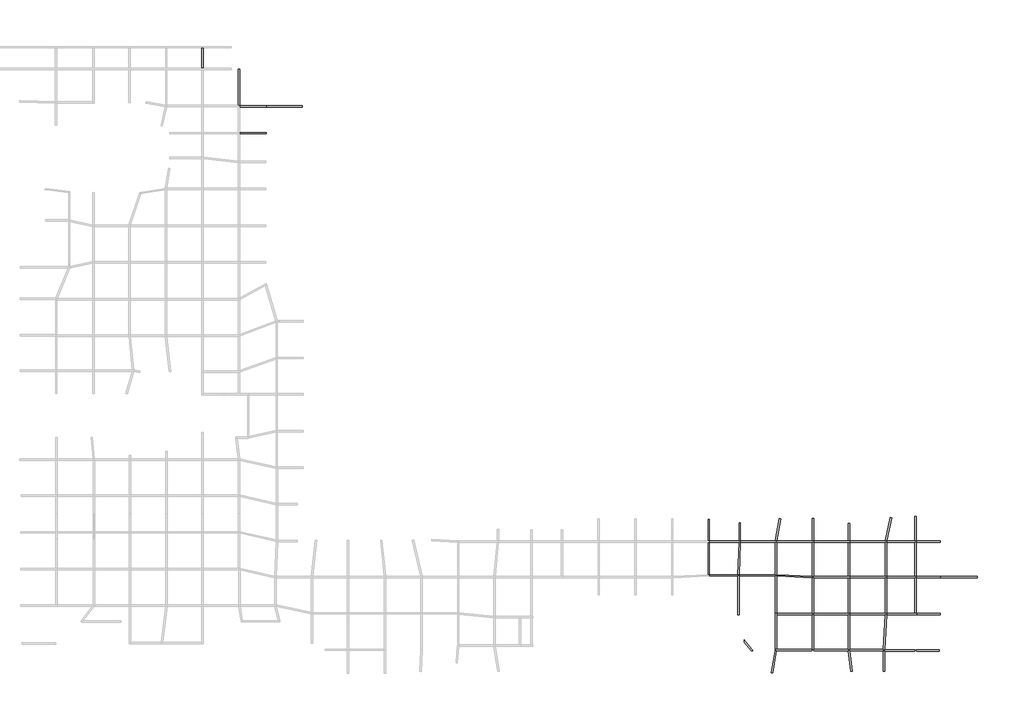
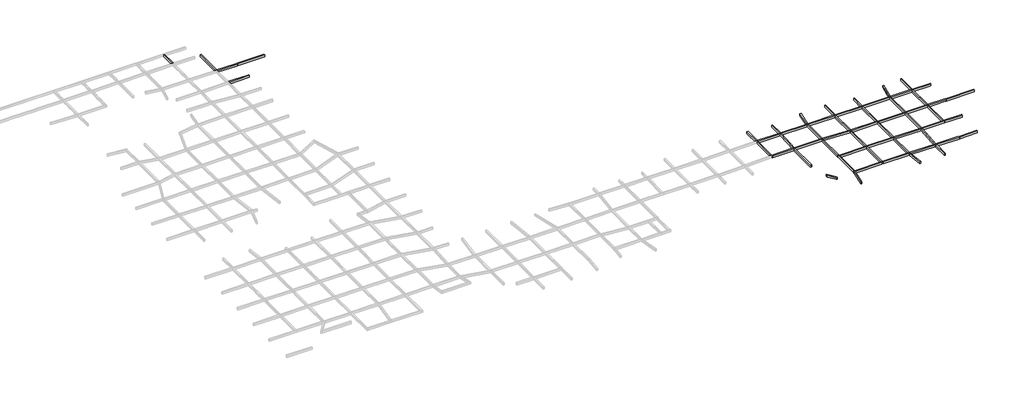
# One storey, part 8 of 8: 58 beams.
"""IFC4 building model written with IfcOpenShell, lengths in millimetres."""

from ifc_helpers import new_model, si_unit, frame, origin, place, context, project, spatial, polyline, outline, extrude, faceted_brep, element, save

model = new_model("IFC4")

# Units and contexts
model_context = context("Model", 3, world=origin())
ifc_project = project(units=[si_unit("LENGTHUNIT", "METRE", prefix="MILLI")], contexts=[model_context])

# Site, building, storey
site = spatial("IfcSite", under=ifc_project)
building = spatial("IfcBuilding", under=site)
storey = spatial("IfcBuildingStorey", under=building, Name="层高", Elevation=3300.0)

# Beams
placement = place(None, origin())
element("IfcBeam", 1, ObjectType="混凝土 - 矩形梁 : KL_beam", at=placement, inside=storey, context=model_context, shape_type="Brep", body=[
    faceted_brep([(149003.4366403, 153267.0451916, 3300.0), (149303.4366403, 153267.0451916, 3300.0), (149303.4366403, 155366.9462381, 3300.0), (149303.4366403, 155766.9462381, 3300.0), (149303.4366403, 157706.8472847, 3300.0), (149003.4366403, 157706.8472847, 3300.0), (149003.4366403, 155766.9462381, 3300.0), (149003.4366403, 155366.9462381, 3300.0), (149003.4366403, 153267.0451916, 2700.0), (149003.4366403, 157706.8472847, 2700.0), (149003.4366403, 155766.9462381, 2700.0), (149003.4366403, 155366.9462381, 2700.0), (149303.4366403, 153267.0451916, 2700.0), (149303.4366403, 157706.8472847, 2700.0), (149303.4366403, 155766.9462381, 2700.0), (149303.4366403, 155366.9462381, 2700.0)], [[[0, 1, 2, 3, 4, 5, 6, 7]], [[8, 0, 7, 6, 5, 9, 10, 11]], [[12, 8, 11, 10, 9, 13, 14, 15]], [[1, 12, 15, 14, 13, 4, 3, 2]], [[1, 0, 8, 12]], [[5, 4, 13, 9]]]),
])
element("IfcBeam", 2, ObjectType="混凝土 - 矩形梁 : KL_beam", at=placement, inside=storey, context=model_context, shape_type="Brep", body=[
    faceted_brep([(265434.4881621, 50816.8475615, 3300.0), (265434.4881621, 51116.8475615, 3300.0), (265134.4881621, 51116.8475615, 3300.0), (258734.4881621, 51116.8475615, 3300.0), (258734.4881621, 50816.8475615, 3300.0), (265129.0414393, 50816.8475615, 3300.0), (265429.2322879, 50816.8475615, 3300.0), (265434.4881621, 50816.8475615, 2700.0), (258734.4881621, 50816.8475615, 2700.0), (265129.0414393, 50816.8475615, 2700.0), (265429.2322879, 50816.8475615, 2700.0), (265434.4881621, 51116.8475615, 2700.0), (258734.4881621, 51116.8475615, 2700.0), (265134.4881621, 51116.8475615, 2700.0)], [[[0, 1, 2, 3, 4, 5, 6]], [[7, 0, 6, 5, 4, 8, 9, 10]], [[11, 7, 10, 9, 8, 12, 13]], [[1, 11, 13, 12, 3, 2]], [[1, 0, 7, 11]], [[4, 3, 12, 8]]]),
])
element("IfcBeam", 3, ObjectType="混凝土 - 矩形梁 : KL_beam", at=placement, inside=storey, context=model_context, shape_type="Brep", body=[
    faceted_brep([(273210.3531067, 50816.8475615, 3300.0), (273263.2512009, 51116.8475615, 3300.0), (272958.6232174, 51116.8475615, 3300.0), (265434.4881621, 51116.8475615, 3300.0), (265434.4881621, 50816.8475615, 3300.0), (272934.4881621, 50816.8475615, 3300.0), (273210.3531067, 50816.8475615, 2700.0), (265434.4881621, 50816.8475615, 2700.0), (272934.4881621, 50816.8475615, 2700.0), (273263.2512009, 51116.8475615, 2700.0), (265434.4881621, 51116.8475615, 2700.0), (272958.6232174, 51116.8475615, 2700.0)], [[[0, 1, 2, 3, 4, 5]], [[6, 0, 5, 4, 7, 8]], [[9, 6, 8, 7, 10, 11]], [[1, 9, 11, 10, 3, 2]], [[1, 0, 6, 9]], [[4, 3, 10, 7]]]),
])
element("IfcBeam", 4, ObjectType="混凝土 - 矩形梁 : KL_beam", at=placement, inside=storey, context=model_context, shape_type="Brep", body=[
    faceted_brep([(281234.4881621, 50816.8475615, 3300.0), (281234.4881621, 51116.8475615, 3300.0), (280934.4881621, 51116.8475615, 3300.0), (273263.2512009, 51116.8475615, 3300.0), (273210.3531067, 50816.8475615, 3300.0), (273234.4881621, 50816.8475615, 3300.0), (280934.4881621, 50816.8475615, 3300.0), (281234.4881621, 50816.8475615, 2700.0), (273210.3531067, 50816.8475615, 2700.0), (273234.4881621, 50816.8475615, 2700.0), (280934.4881621, 50816.8475615, 2700.0), (281234.4881621, 51116.8475615, 2700.0), (273263.2512009, 51116.8475615, 2700.0), (280934.4881621, 51116.8475615, 2700.0)], [[[0, 1, 2, 3, 4, 5, 6]], [[7, 0, 6, 5, 4, 8, 9, 10]], [[11, 7, 10, 9, 8, 12, 13]], [[1, 11, 13, 12, 3, 2]], [[1, 0, 7, 11]], [[4, 3, 12, 8]]]),
])
element("IfcBeam", 5, ObjectType="混凝土 - 矩形梁 : KL_beam", at=placement, inside=storey, context=model_context, shape_type="Brep", body=[
    faceted_brep([(289034.4881621, 50816.8475615, 3300.0), (289034.4881621, 51116.8475615, 3300.0), (288734.4881621, 51116.8475615, 3300.0), (281234.4881621, 51116.8475615, 3300.0), (281234.4881621, 50816.8475615, 3300.0), (288734.4881621, 50816.8475615, 3300.0), (289034.4881621, 50816.8475615, 2700.0), (281234.4881621, 50816.8475615, 2700.0), (288734.4881621, 50816.8475615, 2700.0), (289034.4881621, 51116.8475615, 2700.0), (281234.4881621, 51116.8475615, 2700.0), (288734.4881621, 51116.8475615, 2700.0)], [[[0, 1, 2, 3, 4, 5]], [[6, 0, 5, 4, 7, 8]], [[9, 6, 8, 7, 10, 11]], [[1, 9, 11, 10, 3, 2]], [[4, 3, 10, 7]], [[1, 0, 6, 9]]]),
])
element("IfcBeam", 6, ObjectType="混凝土 - 矩形梁 : KL_beam", at=placement, inside=storey, context=model_context, shape_type="Brep", body=[
    faceted_brep([(297034.4881621, 50816.8475615, 3300.0), (297034.4881621, 51116.8475615, 3300.0), (296763.0205571, 51116.8475615, 3300.0), (289034.4881621, 51116.8475615, 3300.0), (289034.4881621, 50816.8475615, 3300.0), (296734.4881621, 50816.8475615, 3300.0), (297034.4881621, 50816.8475615, 2700.0), (289034.4881621, 50816.8475615, 2700.0), (296734.4881621, 50816.8475615, 2700.0), (297034.4881621, 51116.8475615, 2700.0), (289034.4881621, 51116.8475615, 2700.0), (296763.0205571, 51116.8475615, 2700.0)], [[[0, 1, 2, 3, 4, 5]], [[6, 0, 5, 4, 7, 8]], [[9, 6, 8, 7, 10, 11]], [[1, 9, 11, 10, 3, 2]], [[4, 3, 10, 7]], [[1, 0, 6, 9]]]),
])
element("IfcBeam", 7, ObjectType="混凝土 - 矩形梁 : KL_beam", at=placement, inside=storey, context=model_context, shape_type="Brep", body=[
    faceted_brep([(303434.4881621, 50816.8475615, 3300.0), (303434.4881621, 51116.8475615, 3300.0), (303134.4881621, 51116.8475615, 3300.0), (297069.7227355, 51116.8475615, 3300.0), (297034.4881621, 51116.8475615, 3300.0), (297034.4881621, 50816.8475615, 3300.0), (303134.4881621, 50816.8475615, 3300.0), (303434.4881621, 50816.8475615, 2700.0), (297034.4881621, 50816.8475615, 2700.0), (303134.4881621, 50816.8475615, 2700.0), (303434.4881621, 51116.8475615, 2700.0), (297034.4881621, 51116.8475615, 2700.0), (297069.7227355, 51116.8475615, 2700.0), (303134.4881621, 51116.8475615, 2700.0)], [[[0, 1, 2, 3, 4, 5, 6]], [[7, 0, 6, 5, 8, 9]], [[10, 7, 9, 8, 11, 12, 13]], [[1, 10, 13, 12, 11, 4, 3, 2]], [[5, 4, 11, 8]], [[1, 0, 7, 10]]]),
])
element("IfcBeam", 8, ObjectType="混凝土 - 矩形梁 : KL_beam", at=placement, inside=storey, context=model_context, shape_type="Brep", body=[
    faceted_brep([(308573.5691593, 50816.8475615, 3300.0), (308573.5691593, 51116.8475615, 3300.0), (308273.5691593, 51116.8475615, 3300.0), (303434.4881621, 51116.8475615, 3300.0), (303434.4881621, 50816.8475615, 3300.0), (308273.5691593, 50816.8475615, 3300.0), (308573.5691593, 50816.8475615, 2700.0), (303434.4881621, 50816.8475615, 2700.0), (308273.5691593, 50816.8475615, 2700.0), (308573.5691593, 51116.8475615, 2700.0), (303434.4881621, 51116.8475615, 2700.0), (308273.5691593, 51116.8475615, 2700.0)], [[[0, 1, 2, 3, 4, 5]], [[6, 0, 5, 4, 7, 8]], [[9, 6, 8, 7, 10, 11]], [[1, 9, 11, 10, 3, 2]], [[4, 3, 10, 7]], [[1, 0, 6, 9]]]),
])
element("IfcBeam", 9, ObjectType="混凝土 - 矩形梁 : KL_beam", at=placement, inside=storey, context=model_context, shape_type="SweptSolid", body=[
    extrude(outline(polyline([(280934.4881621, 55914.1029719), (281234.4881621, 55914.1029719), (281234.4881621, 51116.8475615), (280934.4881621, 51116.8475615), (280934.4881621, 55914.1029719)])), frame((0.0, 0.0, 2700.0), z_axis=(0.0, 0.0, 1.0), x_axis=(1.0, 0.0, 0.0)), (0.0, 0.0, 1.0), 600.0),
])
element("IfcBeam", 10, ObjectType="混凝土 - 矩形梁 : KL_beam", at=placement, inside=storey, context=model_context, shape_type="SweptSolid", body=[
    extrude(outline(polyline([(288734.4881621, 54914.1029731), (289034.4881621, 54914.1029731), (289034.4881621, 51116.8475615), (288734.4881621, 51116.8475615), (288734.4881621, 54914.1029731)])), frame((0.0, 0.0, 2700.0), z_axis=(0.0, 0.0, 1.0), x_axis=(1.0, 0.0, 0.0)), (0.0, 0.0, 1.0), 600.0),
])
element("IfcBeam", 11, ObjectType="混凝土 - 矩形梁 : KL_beam", at=placement, inside=storey, context=model_context, shape_type="SweptSolid", body=[
    extrude(outline(polyline([(273809.0742199, 55939.9948703), (274104.5165458, 55887.900417), (273263.2512009, 51116.8475615), (272958.6232174, 51116.8475615), (273809.0742199, 55939.9948703)])), frame((0.0, 0.0, 2700.0), z_axis=(0.0, 0.0, 1.0), x_axis=(1.0, 0.0, 0.0)), (0.0, 0.0, 1.0), 600.0),
])
element("IfcBeam", 12, ObjectType="混凝土 - 矩形梁 : KL_beam", at=placement, inside=storey, context=model_context, shape_type="SweptSolid", body=[
    extrude(outline(polyline([(265134.4881621, 54966.8475615), (265434.4881621, 54966.8475615), (265434.4881621, 51116.8475615), (265134.4881621, 51116.8475615), (265134.4881621, 54966.8475615)])), frame((0.0, 0.0, 2700.0), z_axis=(0.0, 0.0, 1.0), x_axis=(1.0, 0.0, 0.0)), (0.0, 0.0, 1.0), 600.0),
])
element("IfcBeam", 13, ObjectType="混凝土 - 矩形梁 : KL_beam", at=placement, inside=storey, context=model_context, shape_type="SweptSolid", body=[
    extrude(outline(polyline([(258434.4881621, 55766.1863398), (258734.4881621, 55766.1863398), (258734.4881621, 51116.8475615), (258434.4881621, 51116.8475615), (258434.4881621, 55766.1863398)])), frame((0.0, 0.0, 2700.0), z_axis=(0.0, 0.0, 1.0), x_axis=(1.0, 0.0, 0.0)), (0.0, 0.0, 1.0), 600.0),
])
element("IfcBeam", 14, ObjectType="混凝土 - 矩形梁 : KL_beam", at=placement, inside=storey, context=model_context, shape_type="Brep", body=[
    faceted_brep([(156905.5468539, 153066.4947596, 3300.0), (157205.5468539, 153066.4947596, 3300.0), (157205.5468539, 153066.4947596, 2700.0), (156905.5468539, 153066.4947596, 2700.0), (156905.5468539, 150806.6496336, 3300.0), (156905.5468539, 150406.6496336, 3300.0), (156905.5468539, 148054.2446479, 3300.0), (156905.5468539, 147654.2446479, 3300.0), (156905.5468539, 145267.0451916, 3300.0), (156905.5468539, 145218.3398855, 3300.0), (157205.5468539, 145218.3398855, 3300.0), (157205.5468539, 145218.3398855, 2700.0), (157205.5468539, 147654.2446479, 2700.0), (157205.5468539, 148054.2446479, 2700.0), (157205.5468539, 150406.6496336, 2700.0), (157205.5468539, 150806.6496336, 2700.0), (156905.5468539, 145218.3398855, 2700.0), (156905.5468539, 145267.0451916, 2700.0), (156905.5468539, 147654.2446479, 2700.0), (156905.5468539, 148054.2446479, 2700.0), (156905.5468539, 150406.6496336, 2700.0), (156905.5468539, 150806.6496336, 2700.0)], [[[0, 1, 2, 3]], [[1, 0, 4, 5, 6, 7, 8, 9, 10]], [[2, 1, 10, 11, 12, 13, 14, 15]], [[3, 2, 15, 14, 13, 12, 11, 16, 17, 18, 19, 20, 21]], [[0, 3, 21, 20, 19, 18, 17, 16, 9, 8, 7, 6, 5, 4]], [[10, 9, 16, 11]]]),
])
element("IfcBeam", 15, ObjectType="混凝土 - 矩形梁 : KL_beam", at=placement, inside=storey, context=model_context, shape_type="Brep", body=[
    faceted_brep([(163005.5468539, 144918.3398855, 3300.0), (163005.5468539, 145218.3398855, 3300.0), (162705.5468539, 145218.3398855, 3300.0), (157205.5468539, 145218.3398855, 3300.0), (157205.5468539, 144918.3398855, 3300.0), (162705.5468539, 144918.3398855, 3300.0), (163005.5468539, 144918.3398855, 2700.0), (157205.5468539, 144918.3398855, 2700.0), (162705.5468539, 144918.3398855, 2700.0), (163005.5468539, 145218.3398855, 2700.0), (157205.5468539, 145218.3398855, 2700.0), (162705.5468539, 145218.3398855, 2700.0)], [[[0, 1, 2, 3, 4, 5]], [[6, 0, 5, 4, 7, 8]], [[9, 6, 8, 7, 10, 11]], [[1, 9, 11, 10, 3, 2]], [[4, 3, 10, 7]], [[1, 0, 6, 9]]]),
])
element("IfcBeam", 16, ObjectType="混凝土 - 矩形梁 : KL_beam", at=placement, inside=storey, context=model_context, shape_type="Brep", body=[
    faceted_brep([(163005.5468539, 139118.3398855, 3300.0), (163005.5468539, 139418.3398855, 3300.0), (162705.5468539, 139418.3398855, 3300.0), (157205.5468539, 139418.3398855, 3300.0), (157205.5468539, 139118.3398855, 3300.0), (163005.5468539, 139118.3398855, 2700.0), (157205.5468539, 139118.3398855, 2700.0), (163005.5468539, 139418.3398855, 2700.0), (157205.5468539, 139418.3398855, 2700.0), (162705.5468539, 139418.3398855, 2700.0)], [[[0, 1, 2, 3, 4]], [[5, 0, 4, 6]], [[7, 5, 6, 8, 9]], [[1, 7, 9, 8, 3, 2]], [[4, 3, 8, 6]], [[1, 0, 5, 7]]]),
])
element("IfcBeam", 17, ObjectType="混凝土 - 矩形梁 : KL_beam", at=placement, inside=storey, context=model_context, shape_type="SweptSolid", body=[
    extrude(outline(polyline([(170773.6972933, 145218.3398855), (170773.6972933, 144918.3398855), (163005.5468539, 144918.3398855), (163005.5468539, 145218.3398855), (170773.6972933, 145218.3398855)])), frame((0.0, 0.0, 2700.0), z_axis=(0.0, 0.0, 1.0), x_axis=(1.0, 0.0, 0.0)), (0.0, 0.0, 1.0), 600.0),
])
element("IfcBeam", 18, ObjectType="混凝土 - 矩形梁 : KL_beam", at=placement, inside=storey, context=model_context, shape_type="SweptSolid", body=[
    extrude(outline(polyline([(258434.4881621, 50816.8475615), (258734.4881621, 50816.8475615), (258734.4881621, 43805.1468492), (258434.4881621, 43789.4245154), (258434.4881621, 50816.8475615)])), frame((0.0, 0.0, 2700.0), z_axis=(0.0, 0.0, 1.0), x_axis=(1.0, 0.0, 0.0)), (0.0, 0.0, 1.0), 600.0),
])
element("IfcBeam", 19, ObjectType="混凝土 - 矩形梁 : KL_beam", at=placement, inside=storey, context=model_context, shape_type="Brep", body=[
    faceted_brep([(258734.4881621, 43504.7351454, 3300.0), (258588.4160503, 43497.0798304, 3300.0), (258734.4881621, 43497.0798304, 3300.0), (264873.3530817, 43497.0798304, 3300.0), (265168.0972075, 43497.0798304, 3300.0), (265178.7998045, 43797.0798304, 3300.0), (264878.6089559, 43797.0798304, 3300.0), (258734.4881621, 43797.0798304, 3300.0), (258588.4160503, 43497.0798304, 2700.0), (258734.4881621, 43497.0798304, 2700.0), (264873.3530817, 43497.0798304, 2700.0), (265168.0972075, 43497.0798304, 2700.0), (258734.4881621, 43504.7351454, 2700.0), (258734.4881621, 43797.0798304, 2700.0), (264878.6089559, 43797.0798304, 2700.0), (265178.7998045, 43797.0798304, 2700.0)], [[[0, 1, 2, 3, 4, 5, 6, 7]], [[1, 8, 9, 10, 11, 4, 3, 2]], [[8, 12, 13, 14, 15, 11, 10, 9]], [[13, 7, 6, 5, 15, 14]], [[0, 12, 8, 1]], [[12, 0, 7, 13]], [[5, 4, 11, 15]]]),
])
element("IfcBeam", 20, ObjectType="混凝土 - 矩形梁 : KL_beam", at=placement, inside=storey, context=model_context, shape_type="Brep", body=[
    faceted_brep([(265429.2322879, 50816.8475615, 3300.0), (265134.4881621, 50816.8475615, 3300.0), (265129.0414393, 50816.8475615, 3300.0), (264878.6089559, 43797.0798304, 3300.0), (265178.7998045, 43797.0798304, 3300.0), (265129.0414393, 50816.8475615, 2700.0), (264878.6089559, 43797.0798304, 2700.0), (265134.4881621, 50816.8475615, 2700.0), (265429.2322879, 50816.8475615, 2700.0), (265178.7998045, 43797.0798304, 2700.0)], [[[0, 1, 2, 3, 4]], [[2, 5, 6, 3]], [[5, 7, 8, 9, 6]], [[8, 0, 4, 9]], [[5, 2, 1, 0, 8, 7]], [[4, 3, 6, 9]]]),
])
element("IfcBeam", 21, ObjectType="混凝土 - 矩形梁 : KL_beam", at=placement, inside=storey, context=model_context, shape_type="Brep", body=[
    faceted_brep([(273234.4881621, 50816.8475615, 3300.0), (273210.3531067, 50816.8475615, 3300.0), (272934.4881621, 50816.8475615, 3300.0), (272934.4881621, 43797.0798304, 3300.0), (272934.4881621, 43497.0798304, 3300.0), (273080.9254954, 43497.0798304, 3300.0), (273234.4881621, 43497.0798304, 3300.0), (273234.4881621, 43790.1198055, 3300.0), (272934.4881621, 50816.8475615, 2700.0), (272934.4881621, 43797.0798304, 2700.0), (272934.4881621, 43497.0798304, 2700.0), (273210.3531067, 50816.8475615, 2700.0), (273234.4881621, 50816.8475615, 2700.0), (273234.4881621, 43790.1198055, 2700.0), (273234.4881621, 43497.0798304, 2700.0), (273080.9254954, 43497.0798304, 2700.0)], [[[0, 1, 2, 3, 4, 5, 6, 7]], [[2, 8, 9, 10, 4, 3]], [[8, 11, 12, 13, 14, 15, 10, 9]], [[6, 14, 13, 12, 0, 7]], [[0, 12, 11, 8, 2, 1]], [[6, 5, 4, 10, 15, 14]]]),
])
element("IfcBeam", 22, ObjectType="混凝土 - 矩形梁 : KL_beam", at=placement, inside=storey, context=model_context, shape_type="Brep", body=[
    faceted_brep([(265178.7998045, 43797.0798304, 3300.0), (265168.0972075, 43497.0798304, 3300.0), (265173.3530817, 43497.0798304, 3300.0), (272934.4881621, 43497.0798304, 3300.0), (272934.4881621, 43797.0798304, 3300.0), (265168.0972075, 43497.0798304, 2700.0), (265173.3530817, 43497.0798304, 2700.0), (272934.4881621, 43497.0798304, 2700.0), (265178.7998045, 43797.0798304, 2700.0), (272934.4881621, 43797.0798304, 2700.0)], [[[0, 1, 2, 3, 4]], [[1, 5, 6, 7, 3, 2]], [[5, 8, 9, 7, 6]], [[8, 0, 4, 9]], [[1, 0, 8, 5]], [[4, 3, 7, 9]]]),
])
element("IfcBeam", 23, ObjectType="混凝土 - 矩形梁 : KL_beam", at=placement, inside=storey, context=model_context, shape_type="Brep", body=[
    faceted_brep([(280934.4881621, 43123.8075864, 3300.0), (281234.4881621, 43123.8075864, 3300.0), (281234.4881621, 43416.8475615, 3300.0), (281234.4881621, 50816.8475615, 3300.0), (280934.4881621, 50816.8475615, 3300.0), (280934.4881621, 43424.1462466, 3300.0), (280934.4881621, 43123.8075864, 2700.0), (280934.4881621, 50816.8475615, 2700.0), (280934.4881621, 43424.1462466, 2700.0), (281234.4881621, 43123.8075864, 2700.0), (281234.4881621, 50816.8475615, 2700.0), (281234.4881621, 43416.8475615, 2700.0)], [[[0, 1, 2, 3, 4, 5]], [[6, 0, 5, 4, 7, 8]], [[9, 6, 8, 7, 10, 11]], [[1, 9, 11, 10, 3, 2]], [[4, 3, 10, 7]], [[1, 0, 6, 9]]]),
])
element("IfcBeam", 24, ObjectType="混凝土 - 矩形梁 : KL_beam", at=placement, inside=storey, context=model_context, shape_type="Brep", body=[
    faceted_brep([(281234.4881621, 43109.5488763, 3300.0), (281234.4881621, 43116.8475615, 3300.0), (281234.4881621, 43123.8075864, 3300.0), (280934.4881621, 43123.8075864, 3300.0), (281080.9254954, 43116.8475615, 3300.0), (281234.4881621, 43109.5488763, 2700.0), (273234.4881621, 43489.7811453, 3300.0), (273080.9254954, 43497.0798304, 3300.0), (273080.9254954, 43497.0798304, 2700.0), (273234.4881621, 43489.7811453, 2700.0), (280934.4881621, 43123.8075864, 2700.0), (281080.9254954, 43116.8475615, 2700.0), (281234.4881621, 43123.8075864, 2700.0), (281234.4881621, 43116.8475615, 2700.0), (273234.4881621, 43790.1198055, 2700.0), (273234.4881621, 43790.1198055, 3300.0), (280934.4881621, 43424.1462466, 3300.0), (280934.4881621, 43424.1462466, 2700.0), (273234.4881621, 43497.0798304, 2700.0), (273234.4881621, 43497.0798304, 3300.0)], [[[0, 1, 2, 3, 4]], [[5, 0, 4, 3, 6, 7, 8, 9, 10, 11]], [[12, 13, 5, 11, 10]], [[14, 15, 16, 17]], [[0, 5, 13, 12, 2, 1]], [[18, 19, 15, 14]], [[19, 18, 8, 7]], [[3, 10, 17, 16]], [[10, 3, 2, 12]], [[15, 19, 7, 6, 3, 16]], [[18, 14, 17, 10, 9, 8]]]),
])
element("IfcBeam", 25, ObjectType="混凝土 - 矩形梁 : KL_beam", at=placement, inside=storey, context=model_context, shape_type="Brep", body=[
    faceted_brep([(289034.4881621, 43116.8475615, 3300.0), (289034.4881621, 43416.8475615, 3300.0), (288734.4881621, 43416.8475615, 3300.0), (281234.4881621, 43416.8475615, 3300.0), (281234.4881621, 43123.8075864, 3300.0), (281234.4881621, 43116.8475615, 3300.0), (288734.4881621, 43116.8475615, 3300.0), (289034.4881621, 43116.8475615, 2700.0), (281234.4881621, 43116.8475615, 2700.0), (288734.4881621, 43116.8475615, 2700.0), (289034.4881621, 43416.8475615, 2700.0), (281234.4881621, 43123.8075864, 2700.0), (281234.4881621, 43416.8475615, 2700.0), (288734.4881621, 43416.8475615, 2700.0)], [[[0, 1, 2, 3, 4, 5, 6]], [[7, 0, 6, 5, 8, 9]], [[10, 7, 9, 8, 11, 12, 13]], [[12, 3, 2, 1, 10, 13]], [[3, 12, 11, 8, 5, 4]], [[1, 0, 7, 10]]]),
    faceted_brep([(280934.4881621, 43116.8475615, 2700.0), (280934.4881621, 43116.8475615, 3300.0), (280934.4881621, 43123.8075864, 3300.0), (280934.4881621, 43123.8075864, 2700.0), (281080.9254954, 43116.8475615, 3300.0), (281080.9254954, 43116.8475615, 2700.0)], [[[0, 1, 2, 3]], [[2, 4, 5, 3]], [[2, 1, 4]], [[1, 0, 5, 4]], [[0, 3, 5]]]),
])
element("IfcBeam", 26, ObjectType="混凝土 - 矩形梁 : KL_beam", at=placement, inside=storey, context=model_context, shape_type="Brep", body=[
    faceted_brep([(297034.4881621, 43116.8475615, 3300.0), (297034.4881621, 43416.8475615, 3300.0), (296734.4881621, 43416.8475615, 3300.0), (289034.4881621, 43416.8475615, 3300.0), (289034.4881621, 43116.8475615, 3300.0), (296734.4881621, 43116.8475615, 3300.0), (297034.4881621, 43116.8475615, 2700.0), (289034.4881621, 43116.8475615, 2700.0), (296734.4881621, 43116.8475615, 2700.0), (297034.4881621, 43416.8475615, 2700.0), (289034.4881621, 43416.8475615, 2700.0), (296734.4881621, 43416.8475615, 2700.0)], [[[0, 1, 2, 3, 4, 5]], [[6, 0, 5, 4, 7, 8]], [[9, 6, 8, 7, 10, 11]], [[1, 9, 11, 10, 3, 2]], [[4, 3, 10, 7]], [[1, 0, 6, 9]]]),
])
element("IfcBeam", 27, ObjectType="混凝土 - 矩形梁 : KL_beam", at=placement, inside=storey, context=model_context, shape_type="Brep", body=[
    faceted_brep([(303434.4881621, 43116.8475615, 3300.0), (303434.4881621, 43416.8475615, 3300.0), (303134.4881621, 43416.8475615, 3300.0), (297034.4881621, 43416.8475615, 3300.0), (297034.4881621, 43116.8475615, 3300.0), (303134.4881621, 43116.8475615, 3300.0), (303434.4881621, 43116.8475615, 2700.0), (297034.4881621, 43116.8475615, 2700.0), (303134.4881621, 43116.8475615, 2700.0), (303434.4881621, 43416.8475615, 2700.0), (297034.4881621, 43416.8475615, 2700.0), (303134.4881621, 43416.8475615, 2700.0)], [[[0, 1, 2, 3, 4, 5]], [[6, 0, 5, 4, 7, 8]], [[9, 6, 8, 7, 10, 11]], [[1, 9, 11, 10, 3, 2]], [[4, 3, 10, 7]], [[1, 0, 6, 9]]]),
])
element("IfcBeam", 28, ObjectType="混凝土 - 矩形梁 : KL_beam", at=placement, inside=storey, context=model_context, shape_type="Brep", body=[
    faceted_brep([(308573.5691593, 43116.8475615, 3300.0), (308573.5691593, 43416.8475615, 3300.0), (308273.5691593, 43416.8475615, 3300.0), (303434.4881621, 43416.8475615, 3300.0), (303434.4881621, 43116.8475615, 3300.0), (308273.5691593, 43116.8475615, 3300.0), (308573.5691593, 43116.8475615, 2700.0), (303434.4881621, 43116.8475615, 2700.0), (308273.5691593, 43116.8475615, 2700.0), (308573.5691593, 43416.8475615, 2700.0), (303434.4881621, 43416.8475615, 2700.0), (308273.5691593, 43416.8475615, 2700.0)], [[[0, 1, 2, 3, 4, 5]], [[6, 0, 5, 4, 7, 8]], [[9, 6, 8, 7, 10, 11]], [[1, 9, 11, 10, 3, 2]], [[4, 3, 10, 7]], [[1, 0, 6, 9]]]),
])
element("IfcBeam", 29, ObjectType="混凝土 - 矩形梁 : KL_beam", at=placement, inside=storey, context=model_context, shape_type="SweptSolid", body=[
    extrude(outline(polyline([(288734.4881621, 50816.8475615), (289034.4881621, 50816.8475615), (289034.4881621, 43416.8475615), (288734.4881621, 43416.8475615), (288734.4881621, 50816.8475615)])), frame((0.0, 0.0, 2700.0), z_axis=(0.0, 0.0, 1.0), x_axis=(1.0, 0.0, 0.0)), (0.0, 0.0, 1.0), 600.0),
])
element("IfcBeam", 30, ObjectType="混凝土 - 矩形梁 : KL_beam", at=placement, inside=storey, context=model_context, shape_type="SweptSolid", body=[
    extrude(outline(polyline([(296734.4881621, 50816.8475615), (297034.4881621, 50816.8475615), (297034.4881621, 43416.8475615), (296734.4881621, 43416.8475615), (296734.4881621, 50816.8475615)])), frame((0.0, 0.0, 2700.0), z_axis=(0.0, 0.0, 1.0), x_axis=(1.0, 0.0, 0.0)), (0.0, 0.0, 1.0), 600.0),
])
element("IfcBeam", 31, ObjectType="混凝土 - 矩形梁 : KL_beam", at=placement, inside=storey, context=model_context, shape_type="SweptSolid", body=[
    extrude(outline(polyline([(303134.4881621, 50816.8475615), (303434.4881621, 50816.8475615), (303434.4881621, 43416.8475615), (303134.4881621, 43416.8475615), (303134.4881621, 50816.8475615)])), frame((0.0, 0.0, 2700.0), z_axis=(0.0, 0.0, 1.0), x_axis=(1.0, 0.0, 0.0)), (0.0, 0.0, 1.0), 600.0),
])
element("IfcBeam", 32, ObjectType="混凝土 - 矩形梁 : KL_beam", at=placement, inside=storey, context=model_context, shape_type="Brep", body=[
    faceted_brep([(297839.6979833, 56182.216599, 3300.0), (298133.1422635, 56119.8430917, 3300.0), (298133.1422635, 56119.8430917, 2700.0), (297839.6979833, 56182.216599, 2700.0), (296763.0205571, 51116.8475615, 3300.0), (297034.4881621, 51116.8475615, 3300.0), (297069.7227355, 51116.8475615, 3300.0), (297069.7227355, 51116.8475615, 2700.0), (297034.4881621, 51116.8475615, 2700.0), (296763.0205571, 51116.8475615, 2700.0)], [[[0, 1, 2, 3]], [[1, 0, 4, 5, 6]], [[2, 1, 6, 7]], [[3, 2, 7, 8, 9]], [[0, 3, 9, 4]], [[4, 9, 8, 7, 6, 5]]]),
])
element("IfcBeam", 33, ObjectType="混凝土 - 矩形梁 : KL_beam", at=placement, inside=storey, context=model_context, shape_type="SweptSolid", body=[
    extrude(outline(polyline([(303134.4881621, 56414.1029728), (303434.4881621, 56414.1029728), (303434.4881621, 51116.8475615), (303134.4881621, 51116.8475615), (303134.4881621, 56414.1029728)])), frame((0.0, 0.0, 2700.0), z_axis=(0.0, 0.0, 1.0), x_axis=(1.0, 0.0, 0.0)), (0.0, 0.0, 1.0), 600.0),
])
element("IfcBeam", 34, ObjectType="混凝土 - 矩形梁 : KL_beam", at=placement, inside=storey, context=model_context, shape_type="SweptSolid", body=[
    extrude(outline(polyline([(316648.6965569, 43416.8475615), (316648.6965569, 43116.8475615), (308573.5691593, 43116.8475615), (308573.5691593, 43416.8475615), (316648.6965569, 43416.8475615)])), frame((0.0, 0.0, 2700.0), z_axis=(0.0, 0.0, 1.0), x_axis=(1.0, 0.0, 0.0)), (0.0, 0.0, 1.0), 600.0),
])
element("IfcBeam", 35, ObjectType="混凝土 - 矩形梁 : KL_beam", at=placement, inside=storey, context=model_context, shape_type="Brep", body=[
    faceted_brep([(280934.4881621, 35116.8475615, 3300.0), (281234.4881621, 35116.8475615, 3300.0), (281234.4881621, 35416.8475615, 3300.0), (281234.4881621, 43109.5488763, 3300.0), (281080.9254954, 43116.8475615, 3300.0), (280934.4881621, 43116.8475615, 3300.0), (280934.4881621, 35416.8475615, 3300.0), (280934.4881621, 35116.8475615, 2700.0), (280934.4881621, 43116.8475615, 2700.0), (280934.4881621, 35416.8475615, 2700.0), (281234.4881621, 35116.8475615, 2700.0), (281080.9254954, 43116.8475615, 2700.0), (281234.4881621, 43109.5488763, 2700.0), (281234.4881621, 35416.8475615, 2700.0)], [[[0, 1, 2, 3, 4, 5, 6]], [[7, 0, 6, 5, 8, 9]], [[10, 7, 9, 8, 11, 12, 13]], [[12, 3, 2, 1, 10, 13]], [[3, 12, 11, 4]], [[5, 4, 11, 8]], [[1, 0, 7, 10]]]),
])
element("IfcBeam", 36, ObjectType="混凝土 - 矩形梁 : KL_beam", at=placement, inside=storey, context=model_context, shape_type="Brep", body=[
    faceted_brep([(289034.4881621, 35116.8475615, 3300.0), (289034.4881621, 35416.8475615, 3300.0), (288734.4881621, 35416.8475615, 3300.0), (281234.4881621, 35416.8475615, 3300.0), (281234.4881621, 35116.8475615, 3300.0), (288734.4881621, 35116.8475615, 3300.0), (289034.4881621, 35116.8475615, 2700.0), (281234.4881621, 35116.8475615, 2700.0), (288734.4881621, 35116.8475615, 2700.0), (289034.4881621, 35416.8475615, 2700.0), (281234.4881621, 35416.8475615, 2700.0), (288734.4881621, 35416.8475615, 2700.0)], [[[0, 1, 2, 3, 4, 5]], [[6, 0, 5, 4, 7, 8]], [[9, 6, 8, 7, 10, 11]], [[1, 9, 11, 10, 3, 2]], [[4, 3, 10, 7]], [[1, 0, 6, 9]]]),
])
element("IfcBeam", 37, ObjectType="混凝土 - 矩形梁 : KL_beam", at=placement, inside=storey, context=model_context, shape_type="Brep", body=[
    faceted_brep([(297034.4881621, 35116.8475615, 3300.0), (297034.4881621, 35416.8475615, 3300.0), (296734.4881621, 35416.8475615, 3300.0), (289034.4881621, 35416.8475615, 3300.0), (289034.4881621, 35116.8475615, 3300.0), (296726.4211433, 35116.8475615, 3300.0), (297026.8328471, 35116.8475615, 3300.0), (297034.4881621, 35116.8475615, 2700.0), (289034.4881621, 35116.8475615, 2700.0), (296726.4211433, 35116.8475615, 2700.0), (297026.8328471, 35116.8475615, 2700.0), (297034.4881621, 35416.8475615, 2700.0), (289034.4881621, 35416.8475615, 2700.0), (296734.4881621, 35416.8475615, 2700.0)], [[[0, 1, 2, 3, 4, 5, 6]], [[7, 0, 6, 5, 4, 8, 9, 10]], [[11, 7, 10, 9, 8, 12, 13]], [[1, 11, 13, 12, 3, 2]], [[1, 0, 7, 11]], [[4, 3, 12, 8]]]),
])
element("IfcBeam", 38, ObjectType="混凝土 - 矩形梁 : KL_beam", at=placement, inside=storey, context=model_context, shape_type="Brep", body=[
    faceted_brep([(303498.8477341, 35116.8475615, 3300.0), (303498.8477341, 35416.8475615, 3300.0), (303434.4881621, 35416.8475615, 3300.0), (303134.4881621, 35416.8475615, 3300.0), (297034.4881621, 35416.8475615, 3300.0), (297034.4881621, 35116.8475615, 3300.0), (303134.4881621, 35116.8475615, 3300.0), (303434.4881621, 35116.8475615, 3300.0), (303498.8477341, 35116.8475615, 2700.0), (297034.4881621, 35116.8475615, 2700.0), (303134.4881621, 35116.8475615, 2700.0), (303434.4881621, 35116.8475615, 2700.0), (303498.8477341, 35416.8475615, 2700.0), (297034.4881621, 35416.8475615, 2700.0), (303134.4881621, 35416.8475615, 2700.0), (303434.4881621, 35416.8475615, 2700.0)], [[[0, 1, 2, 3, 4, 5, 6, 7]], [[8, 0, 7, 6, 5, 9, 10, 11]], [[12, 8, 11, 10, 9, 13, 14, 15]], [[1, 12, 15, 14, 13, 4, 3, 2]], [[1, 0, 8, 12]], [[5, 4, 13, 9]]]),
])
element("IfcBeam", 39, ObjectType="混凝土 - 矩形梁 : KL_beam", at=placement, inside=storey, context=model_context, shape_type="Brep", body=[
    faceted_brep([(303498.8477341, 35416.8475615, 3300.0), (303498.8477341, 35116.8475615, 3300.0), (308573.5691593, 35116.8475615, 3300.0), (308573.5691593, 35416.8475615, 3300.0), (308273.5691593, 35416.8475615, 3300.0), (303498.8477341, 35116.8475615, 2700.0), (308573.5691593, 35116.8475615, 2700.0), (303498.8477341, 35416.8475615, 2700.0), (308273.5691593, 35416.8475615, 2700.0), (308573.5691593, 35416.8475615, 2700.0)], [[[0, 1, 2, 3, 4]], [[1, 5, 6, 2]], [[5, 7, 8, 9, 6]], [[7, 0, 4, 3, 9, 8]], [[0, 7, 5, 1]], [[3, 2, 6, 9]]]),
])
element("IfcBeam", 40, ObjectType="混凝土 - 矩形梁 : KL_beam", at=placement, inside=storey, context=model_context, shape_type="SweptSolid", body=[
    extrude(outline(polyline([(296734.4881621, 43116.8475615), (297034.4881621, 43116.8475615), (297034.4881621, 35416.8475615), (296734.4881621, 35416.8475615), (296734.4881621, 43116.8475615)])), frame((0.0, 0.0, 2700.0), z_axis=(0.0, 0.0, 1.0), x_axis=(1.0, 0.0, 0.0)), (0.0, 0.0, 1.0), 600.0),
])
element("IfcBeam", 41, ObjectType="混凝土 - 矩形梁 : KL_beam", at=placement, inside=storey, context=model_context, shape_type="SweptSolid", body=[
    extrude(outline(polyline([(288734.4881621, 43116.8475615), (289034.4881621, 43116.8475615), (289034.4881621, 35416.8475615), (288734.4881621, 35416.8475615), (288734.4881621, 43116.8475615)])), frame((0.0, 0.0, 2700.0), z_axis=(0.0, 0.0, 1.0), x_axis=(1.0, 0.0, 0.0)), (0.0, 0.0, 1.0), 600.0),
])
element("IfcBeam", 42, ObjectType="混凝土 - 矩形梁 : KL_beam", at=placement, inside=storey, context=model_context, shape_type="SweptSolid", body=[
    extrude(outline(polyline([(303134.4881621, 43116.8475615), (303434.4881621, 43116.8475615), (303434.4881621, 35416.8475615), (303134.4881621, 35416.8475615), (303134.4881621, 43116.8475615)])), frame((0.0, 0.0, 2700.0), z_axis=(0.0, 0.0, 1.0), x_axis=(1.0, 0.0, 0.0)), (0.0, 0.0, 1.0), 600.0),
])
element("IfcBeam", 43, ObjectType="混凝土 - 矩形梁 : KL_beam", at=placement, inside=storey, context=model_context, shape_type="Brep", body=[
    faceted_brep([(296613.3787927, 27227.6742369, 3300.0), (296629.1011265, 27527.6742369, 3300.0), (297026.8328471, 35116.8475615, 3300.0), (296734.4881621, 35116.8475615, 3300.0), (296726.4211433, 35116.8475615, 3300.0), (296333.3627986, 27616.8475615, 3300.0), (296328.8148297, 27530.0671452, 3300.0), (296321.0341077, 27381.6021251, 3300.0), (296317.6404649, 27316.8475615, 3300.0), (296313.7899323, 27243.3750238, 3300.0), (296726.4211433, 35116.8475615, 2700.0), (296333.3627986, 27616.8475615, 2700.0), (296328.8148297, 27530.0671452, 2700.0), (296321.0341077, 27381.6021251, 2700.0), (296317.6404649, 27316.8475615, 2700.0), (296313.7899323, 27243.3750238, 2700.0), (296734.4881621, 35116.8475615, 2700.0), (297026.8328471, 35116.8475615, 2700.0), (296629.1011265, 27527.6742369, 2700.0), (296613.3787927, 27227.6742369, 2700.0)], [[[0, 1, 2, 3, 4, 5, 6, 7, 8, 9]], [[9, 8, 7, 6, 5, 4, 10, 11, 12, 13, 14, 15]], [[15, 14, 13, 12, 11, 10, 16, 17, 18, 19]], [[2, 1, 0, 19, 18, 17]], [[10, 4, 3, 2, 17, 16]], [[0, 9, 15, 19]]]),
])
element("IfcBeam", 44, ObjectType="混凝土 - 矩形梁 : KL_beam", at=placement, inside=storey, context=model_context, shape_type="Brep", body=[
    faceted_brep([(296629.1011265, 27527.6742369, 3300.0), (296613.3787927, 27227.6742369, 3300.0), (296621.0341077, 27227.6742369, 3300.0), (303102.6187017, 27227.6742369, 3300.0), (303062.8601522, 27527.6742369, 3300.0), (296312.9670889, 27227.6742369, 3300.0), (296312.9670889, 27227.6742369, 2700.0), (296321.0341077, 27227.6742369, 2700.0), (296613.3787927, 27227.6742369, 2700.0), (296621.0341077, 27227.6742369, 2700.0), (303102.6187017, 27227.6742369, 2700.0), (296321.0341077, 27227.6742369, 3300.0), (296629.1011265, 27527.6742369, 2700.0), (303062.8601522, 27527.6742369, 2700.0), (296313.7899323, 27243.3750238, 3300.0), (296313.7899323, 27243.3750238, 2700.0)], [[[0, 1, 2, 3, 4]], [[5, 6, 7, 8, 9, 10, 3, 2, 1, 11]], [[8, 12, 13, 10, 9]], [[12, 0, 4, 13]], [[6, 5, 14, 15]], [[8, 1, 0, 12]], [[1, 8, 15, 14]], [[14, 5, 11, 1]], [[6, 15, 8, 7]], [[4, 3, 10, 13]]]),
])
element("IfcBeam", 45, ObjectType="混凝土 - 矩形梁 : KL_beam", at=placement, inside=storey, context=model_context, shape_type="SweptSolid", body=[
    extrude(outline(polyline([(308423.5286607, 27527.6742369), (308423.5286607, 27227.6742369), (303506.116172, 27227.6742369), (303466.3576224, 27527.6742369), (308423.5286607, 27527.6742369)])), frame((0.0, 0.0, 2700.0), z_axis=(0.0, 0.0, 1.0), x_axis=(1.0, 0.0, 0.0)), (0.0, 0.0, 1.0), 600.0),
])
element("IfcBeam", 46, ObjectType="混凝土 - 矩形梁 : KL_beam", at=placement, inside=storey, context=model_context, shape_type="Brep", body=[
    faceted_brep([(296621.0341077, 22906.8161675, 3300.0), (296321.0341077, 22906.8161675, 3300.0), (296321.0341077, 22906.8161675, 2700.0), (296621.0341077, 22906.8161675, 2700.0), (296621.0341077, 27227.6742369, 3300.0), (296613.3787927, 27227.6742369, 3300.0), (296321.0341077, 27227.6742369, 3300.0), (296321.0341077, 27227.6742369, 2700.0), (296613.3787927, 27227.6742369, 2700.0), (296621.0341077, 27227.6742369, 2700.0)], [[[0, 1, 2, 3]], [[1, 0, 4, 5, 6]], [[2, 1, 6, 7]], [[3, 2, 7, 8, 9]], [[0, 3, 9, 4]], [[5, 4, 9, 8, 7, 6]]]),
    faceted_brep([(296321.0341077, 27530.0671452, 2700.0), (296321.0341077, 27530.0671452, 3300.0), (296328.8148297, 27530.0671452, 3300.0), (296328.8148297, 27530.0671452, 2700.0), (296321.0341077, 27381.6021251, 3300.0), (296321.0341077, 27381.6021251, 2700.0), (296328.6894227, 27527.6742369, 2700.0), (296328.6894227, 27527.6742369, 3300.0)], [[[0, 1, 2, 3]], [[4, 5, 6, 3, 2, 7]], [[2, 1, 4, 7]], [[1, 0, 5, 4]], [[5, 0, 3, 6]]]),
])
element("IfcBeam", 47, ObjectType="混凝土 - 矩形梁 : KL_beam", at=placement, inside=storey, context=model_context, shape_type="Brep", body=[
    faceted_brep([(288734.4881621, 27316.8475615, 3300.0), (288751.7793724, 27316.8475615, 3300.0), (289034.4881621, 27316.8475615, 3300.0), (289034.4881621, 27616.8475615, 3300.0), (289034.4881621, 35116.8475615, 3300.0), (288734.4881621, 35116.8475615, 3300.0), (288734.4881621, 27616.8475615, 3300.0), (288734.4881621, 27316.8475615, 2700.0), (288734.4881621, 35116.8475615, 2700.0), (288734.4881621, 27616.8475615, 2700.0), (289034.4881621, 27316.8475615, 2700.0), (288751.7793724, 27316.8475615, 2700.0), (289034.4881621, 35116.8475615, 2700.0), (289034.4881621, 27616.8475615, 2700.0)], [[[0, 1, 2, 3, 4, 5, 6]], [[7, 0, 6, 5, 8, 9]], [[10, 11, 7, 9, 8, 12, 13]], [[2, 10, 13, 12, 4, 3]], [[5, 4, 12, 8]], [[2, 1, 0, 7, 11, 10]]]),
])
element("IfcBeam", 48, ObjectType="混凝土 - 矩形梁 : KL_beam", at=placement, inside=storey, context=model_context, shape_type="Brep", body=[
    faceted_brep([(296317.6404649, 27316.8475615, 3300.0), (296321.0341077, 27381.6021251, 3300.0), (296321.0341077, 27530.0671452, 3300.0), (296328.8148297, 27530.0671452, 3300.0), (296333.3627986, 27616.8475615, 3300.0), (289034.4881621, 27616.8475615, 3300.0), (289034.4881621, 27316.8475615, 3300.0), (289054.03232, 27316.8475615, 3300.0), (296317.6404649, 27316.8475615, 2700.0), (289034.4881621, 27316.8475615, 2700.0), (289054.03232, 27316.8475615, 2700.0), (296333.3627986, 27616.8475615, 2700.0), (296328.8148297, 27530.0671452, 2700.0), (296321.0341077, 27530.0671452, 2700.0), (296321.0341077, 27381.6021251, 2700.0), (289034.4881621, 27616.8475615, 2700.0)], [[[0, 1, 2, 3, 4, 5, 6, 7]], [[8, 0, 7, 6, 9, 10]], [[11, 12, 13, 14, 8, 10, 9, 15]], [[4, 11, 15, 5]], [[0, 8, 14, 1]], [[13, 2, 1, 14]], [[2, 13, 12, 3]], [[11, 4, 3, 12]], [[6, 5, 15, 9]]]),
])
element("IfcBeam", 49, ObjectType="混凝土 - 矩形梁 : KL_beam", at=placement, inside=storey, context=model_context, shape_type="SweptSolid", body=[
    extrude(outline(polyline([(280934.4881621, 35116.8475615), (281234.4881621, 35116.8475615), (281234.4881621, 27616.8475615), (280934.4881621, 27616.8475615), (280934.4881621, 35116.8475615)])), frame((0.0, 0.0, 2700.0), z_axis=(0.0, 0.0, 1.0), x_axis=(1.0, 0.0, 0.0)), (0.0, 0.0, 1.0), 600.0),
])
element("IfcBeam", 50, ObjectType="混凝土 - 矩形梁 : KL_beam", at=placement, inside=storey, context=model_context, shape_type="SweptSolid", body=[
    extrude(outline(polyline([(288734.4881621, 27616.8475615), (288734.4881621, 27316.8475615), (281284.4881621, 27316.8475615), (281284.4881621, 27616.8475615), (288734.4881621, 27616.8475615)])), frame((0.0, 0.0, 2700.0), z_axis=(0.0, 0.0, 1.0), x_axis=(1.0, 0.0, 0.0)), (0.0, 0.0, 1.0), 600.0),
])
element("IfcBeam", 51, ObjectType="混凝土 - 矩形梁 : KL_beam", at=placement, inside=storey, context=model_context, shape_type="Brep", body=[
    faceted_brep([(272934.4881621, 27616.8475615, 3300.0), (272934.4881621, 27479.970861, 3300.0), (272934.4881621, 27316.8475615, 3300.0), (273210.3531067, 27316.8475615, 3300.0), (280884.4881621, 27316.8475615, 3300.0), (280884.4881621, 27616.8475615, 3300.0), (273234.4881621, 27616.8475615, 3300.0), (272934.4881621, 27616.8475615, 2700.0), (280884.4881621, 27616.8475615, 2700.0), (273234.4881621, 27616.8475615, 2700.0), (272934.4881621, 27316.8475615, 2700.0), (272934.4881621, 27479.970861, 2700.0), (280884.4881621, 27316.8475615, 2700.0), (273210.3531067, 27316.8475615, 2700.0)], [[[0, 1, 2, 3, 4, 5, 6]], [[7, 0, 6, 5, 8, 9]], [[10, 11, 7, 9, 8, 12, 13]], [[2, 10, 13, 12, 4, 3]], [[2, 1, 0, 7, 11, 10]], [[5, 4, 12, 8]]]),
])
element("IfcBeam", 52, ObjectType="混凝土 - 矩形梁 : KL_beam", at=placement, inside=storey, context=model_context, shape_type="Brep", body=[
    faceted_brep([(273234.4881621, 35416.8475615, 3300.0), (272934.4881621, 35416.8475615, 3300.0), (272934.4881621, 35141.452007, 3300.0), (272934.4881621, 27616.8475615, 3300.0), (273234.4881621, 27616.8475615, 3300.0), (273234.4881621, 35116.8475615, 3300.0), (273234.4881621, 35416.8475615, 2700.0), (273234.4881621, 27616.8475615, 2700.0), (273234.4881621, 35116.8475615, 2700.0), (272934.4881621, 35416.8475615, 2700.0), (272934.4881621, 27616.8475615, 2700.0), (272934.4881621, 35141.452007, 2700.0)], [[[0, 1, 2, 3, 4, 5]], [[6, 0, 5, 4, 7, 8]], [[9, 6, 8, 7, 10, 11]], [[1, 9, 11, 10, 3, 2]], [[1, 0, 6, 9]], [[4, 3, 10, 7]]]),
])
element("IfcBeam", 53, ObjectType="混凝土 - 矩形梁 : KL_beam", at=placement, inside=storey, context=model_context, shape_type="SweptSolid", body=[
    extrude(outline(polyline([(280934.4881621, 35416.8475615), (280934.4881621, 35116.8475615), (273234.4881621, 35116.8475615), (273234.4881621, 35416.8475615), (280934.4881621, 35416.8475615)])), frame((0.0, 0.0, 2700.0), z_axis=(0.0, 0.0, 1.0), x_axis=(1.0, 0.0, 0.0)), (0.0, 0.0, 1.0), 600.0),
])
element("IfcBeam", 54, ObjectType="混凝土 - 矩形梁 : KL_beam", at=placement, inside=storey, context=model_context, shape_type="Brep", body=[
    faceted_brep([(273080.9254954, 43497.0798304, 3300.0), (272934.4881621, 43497.0798304, 3300.0), (272934.4881621, 35441.452007, 3300.0), (272934.4881621, 35416.8475615, 3300.0), (273234.4881621, 35416.8475615, 3300.0), (273234.4881621, 43489.7811453, 3300.0), (272934.4881621, 43497.0798304, 2700.0), (272934.4881621, 35441.452007, 2700.0), (272934.4881621, 35416.8475615, 2700.0), (273080.9254954, 43497.0798304, 2700.0), (273234.4881621, 43489.7811453, 2700.0), (273234.4881621, 35416.8475615, 2700.0)], [[[0, 1, 2, 3, 4, 5]], [[1, 6, 7, 8, 3, 2]], [[6, 9, 10, 11, 8, 7]], [[10, 5, 4, 11]], [[6, 1, 0, 9]], [[0, 5, 10, 9]], [[4, 3, 8, 11]]]),
])
element("IfcBeam", 55, ObjectType="混凝土 - 矩形梁 : KL_beam", at=placement, inside=storey, context=model_context, shape_type="Brep", body=[
    faceted_brep([(265173.3530817, 43497.0798304, 3300.0), (265168.0972075, 43497.0798304, 3300.0), (264873.3530817, 43497.0798304, 3300.0), (264873.3530817, 35441.452007, 3300.0), (264873.3530817, 35141.452007, 3300.0), (265173.3530817, 35141.452007, 3300.0), (265173.3530817, 35441.452007, 3300.0), (264873.3530817, 43497.0798304, 2700.0), (264873.3530817, 35441.452007, 2700.0), (264873.3530817, 35141.452007, 2700.0), (265168.0972075, 43497.0798304, 2700.0), (265173.3530817, 43497.0798304, 2700.0), (265173.3530817, 35441.452007, 2700.0), (265173.3530817, 35141.452007, 2700.0)], [[[0, 1, 2, 3, 4, 5, 6]], [[2, 7, 8, 9, 4, 3]], [[7, 10, 11, 12, 13, 9, 8]], [[5, 13, 12, 11, 0, 6]], [[0, 11, 10, 7, 2, 1]], [[5, 4, 9, 13]]]),
])
element("IfcBeam", 56, ObjectType="混凝土 - 矩形梁 : KL_beam", at=placement, inside=storey, context=model_context, shape_type="Brep", body=[
    faceted_brep([(267712.428377, 27316.8475615, 3300.0), (268088.7951021, 27316.8475615, 3300.0), (267861.5245326, 27616.8475615, 3300.0), (266573.353082, 29317.2500198, 3300.0), (266273.353082, 29713.2537795, 3300.0), (266273.353082, 29216.4449856, 3300.0), (267712.428377, 27316.8475615, 2700.0), (266273.353082, 29216.4449856, 2700.0), (268088.7951021, 27316.8475615, 2700.0), (266273.353082, 29713.2537795, 2700.0), (266573.353082, 29317.2500198, 2700.0), (267861.5245326, 27616.8475615, 2700.0)], [[[0, 1, 2, 3, 4, 5]], [[6, 0, 5, 7]], [[8, 6, 7, 9, 10, 11]], [[1, 8, 11, 10, 9, 4, 3, 2]], [[1, 0, 6, 8]], [[5, 4, 9, 7]]]),
])
element("IfcBeam", 57, ObjectType="混凝土 - 矩形梁 : KL_beam", at=placement, inside=storey, context=model_context, shape_type="Brep", body=[
    faceted_brep([(289593.2540515, 22925.238979, 3300.0), (289295.490206, 22888.678176, 3300.0), (289295.490206, 22888.678176, 2700.0), (289593.2540515, 22925.238979, 2700.0), (289054.03232, 27316.8475615, 3300.0), (289034.4881621, 27316.8475615, 3300.0), (288751.7793724, 27316.8475615, 3300.0), (288751.7793724, 27316.8475615, 2700.0), (289034.4881621, 27316.8475615, 2700.0), (289054.03232, 27316.8475615, 2700.0)], [[[0, 1, 2, 3]], [[1, 0, 4, 5, 6]], [[2, 1, 6, 7]], [[3, 2, 7, 8, 9]], [[0, 3, 9, 4]], [[7, 6, 5, 4, 9, 8]]]),
])
element("IfcBeam", 58, ObjectType="混凝土 - 矩形梁 : KL_beam", at=placement, inside=storey, context=model_context, shape_type="Brep", body=[
    faceted_brep([(272371.0530132, 22556.9402, 3300.0), (272075.6106873, 22609.0346533, 3300.0), (272075.6106873, 22609.0346533, 2700.0), (272371.0530132, 22556.9402, 2700.0), (273210.3531067, 27316.8475615, 3300.0), (272934.4881621, 27316.8475615, 3300.0), (272934.4881621, 27479.970861, 3300.0), (272905.7251232, 27316.8475615, 3300.0), (272934.4881621, 27479.970861, 2700.0), (272905.7251232, 27316.8475615, 2700.0), (272934.4881621, 27316.8475615, 2700.0), (273210.3531067, 27316.8475615, 2700.0)], [[[0, 1, 2, 3]], [[1, 0, 4, 5, 6, 7]], [[2, 1, 7, 6, 8, 9]], [[3, 2, 9, 8, 10, 11]], [[0, 3, 11, 4]], [[5, 4, 11, 10]], [[5, 10, 8, 6]]]),
])

save(model, "model.ifc")

# Revit data of these elements
# Type "混凝土 - 矩形梁 : KL_beam"
#   Length [instance default] = 1524 mm
#   b = 300 mm
#   h = 600 mm
#   Structural Material [instance default] = 混凝土 - 现场浇注混凝土
#   Assembly Code = ""
# Elements 1, 2, 3, 4, 5, 6, 7, 8, 9, 10, 11, 12, 13, 14, 15, 16, 17, 18, 19, 20, 21, 22, 23, 24, 25, 26, 27, 28, 29, 30, 31, 32, 33, 34, 35, 36, 37, 38, 39, 40, 41, 42, 43, 44, 45, 46, 47, 48, 49, 50, 51, 52, 53, 54, 55, 56, 57, 58 (IfcBeam, "混凝土 - 矩形梁 : KL_beam")
#   Comments = ""
#   Structural Material = none
#   Phase Created = 新构造
# Materials
#   "混凝土 - 现场浇注混凝土": class "混凝土", colour RGB 192 192 192, transparency 0
